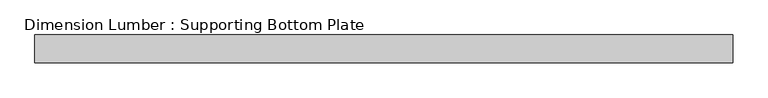
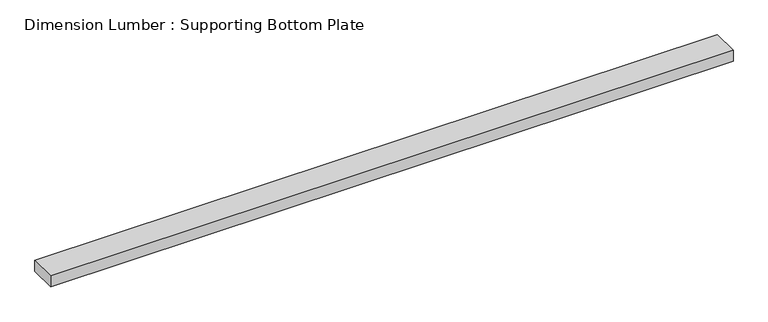
"""IFC4 building model written with IfcOpenShell, lengths in millimetres: beam geometry, Dimension Lumber : Supporting Bottom Plate."""

from ifc_helpers import new_model, si_unit, frame, origin, place, context, project, spatial, polyline, outline, extrude, source, transform, mapped, element, save


def dimension_lumber_supporting_bottom_plate_4a764e13(model_context):
    return source(origin(), model_context, "Body", "SweptSolid", [
        extrude(outline(polyline([(316.70625, -44.45), (-1918.49375, -44.45), (-1918.49375, 44.45), (316.70625, 44.45), (316.70625, -44.45)])), frame((0.0, 0.0, -19.05), z_axis=(0.0, 0.0, 1.0), x_axis=(1.0, 0.0, 0.0)), (0.0, 0.0, 1.0), 38.1),
    ])


if __name__ == "__main__":
    model = new_model("IFC4")
    model_context = context("Model", 3, world=origin())
    ifc_project = project(units=[si_unit("LENGTHUNIT", "METRE", prefix="MILLI")], contexts=[model_context])
    site = spatial("IfcSite", under=ifc_project)
    building = spatial("IfcBuilding", under=site)
    placement = place(None, origin())
    dimension_lumber_supporting_bottom_plate_shape = dimension_lumber_supporting_bottom_plate_4a764e13(model_context)
    element("IfcBeam", 1, ObjectType="Dimension Lumber : Supporting Bottom Plate", at=placement, inside=building, context=model_context, shape_type="MappedRepresentation", body=[
        mapped(dimension_lumber_supporting_bottom_plate_shape, transform((0.0, 0.0, 0.0), x_axis=(1.0, 0.0, 0.0), y_axis=(0.0, 1.0, 0.0), z_axis=(0.0, 0.0, 1.0))),
    ])
    save(model, "model.ifc")

# Revit data of these elements
# Type "Dimension Lumber : Supporting Bottom Plate"
#   Assembly Code = "B10"
#   A = 0.0364583 SF
#   Length [instance default] = 5' - 0"
#   b = 0' - 3 1/2"
#   d = 0' - 1 1/2"
#   Structural Material [instance default] = Softwood, Lumber
# Element 1 (IfcBeam, "Dimension Lumber : Supporting Bottom Plate")
#   Structural Material = Douglas Fir #2
#   Materials on its faces: "Douglas Fir #2"
# Materials
#   "Softwood, Lumber": class "Wood", colour RGB 223 192 134, transparency 0, Description = "Pinus Echinata", Cost = 0
#   "Douglas Fir #2": class "Wood", colour RGB 223 192 134, transparency 0, Description = "Pinus Echinata", Cost = 0
